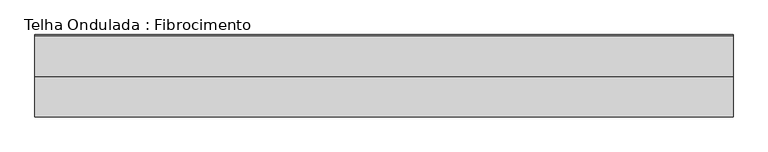
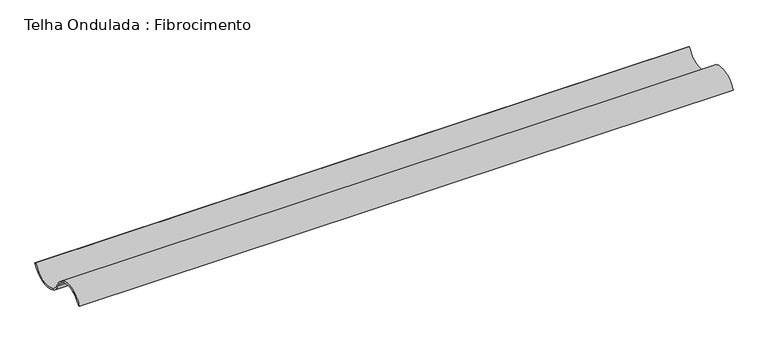
"""IFC4 building model written with IfcOpenShell, lengths in millimetres: beam geometry, Telha Ondulada : Fibrocimento."""

from ifc_helpers import new_model, si_unit, point, frame, frame_2d, origin, place, context, project, spatial, polyline, circle_curve, trimmed, segment, composite_curve, outline, extrude, source, transform, mapped, element, save


def telha_ondulada_fibrocimento_69359d52(model_context):
    return source(origin(), model_context, "Body", "SweptSolid", [
        extrude(outline(composite_curve([segment(trimmed(circle_curve(frame_2d((68.3970135, 71.7939461)), 66.7939461), [point((8.3970135, 42.4437972))], [point((128.3970135, 42.4437972))], True, "CARTESIAN"), True, "CONTINUOUS"), segment(polyline([(128.3970135, 42.4437972), (132.8884385, 40.2467307)]), True, "CONTINUOUS"), segment(trimmed(circle_curve(frame_2d((68.3970135, 71.7939461)), 71.7939461), [point((132.8884385, 40.2467307))], [point((3.9055884, 40.2467307))], False, "CARTESIAN"), True, "CONTINUOUS"), segment(trimmed(circle_curve(frame_2d((-51.6029865, 13.0936483)), 61.7939461), [point((3.9055884, 40.2467307))], [point((-107.1115615, 40.2467307))], True, "CARTESIAN"), True, "CONTINUOUS"), segment(polyline([(-107.1115615, 40.2467307), (-111.6029865, 42.4437972)]), True, "CONTINUOUS"), segment(trimmed(circle_curve(frame_2d((-51.6029865, 13.0936483)), 66.7939461), [point((-111.6029865, 42.4437972))], [point((8.3970135, 42.4437972))], False, "CARTESIAN"), True, "CONTINUOUS")], self_intersect=False)), frame((-1038.2805783, 0.0, 0.0), z_axis=(1.0, 0.0, 0.0), x_axis=(0.0, 1.0, 0.0)), (0.0, 0.0, 1.0), 2076.5611566),
    ])


if __name__ == "__main__":
    model = new_model("IFC4")
    model_context = context("Model", 3, world=origin())
    ifc_project = project(units=[si_unit("LENGTHUNIT", "METRE", prefix="MILLI")], contexts=[model_context])
    site = spatial("IfcSite", under=ifc_project)
    building = spatial("IfcBuilding", under=site)
    placement = place(None, origin())
    telha_ondulada_fibrocimento_shape = telha_ondulada_fibrocimento_69359d52(model_context)
    element("IfcBeam", 1, ObjectType="Telha Ondulada : Fibrocimento", at=placement, inside=building, context=model_context, shape_type="MappedRepresentation", body=[
        mapped(telha_ondulada_fibrocimento_shape, transform((0.0, 0.0, 0.0), x_axis=(1.0, 0.0, 0.0), y_axis=(0.0, 1.0, 0.0), z_axis=(0.0, 0.0, 1.0))),
    ])
    save(model, "model.ifc")

# Revit data of these elements
# Type "Telha Ondulada : Fibrocimento"
#   Description = "TELHA ONDULADA FIBROCIMENTO"
#   Cost = 5
#   Length [instance default] = 1.524 m
#   b = 0.07 m
#   h = 0.16 m
#   Structural Material = .TELHA DE FIBROCIMENTO
#   Assembly Code = ""
# Element 1 (IfcBeam, "Telha Ondulada : Fibrocimento")
#   Materials on its faces: ".TELHA DE FIBROCIMENTO"
# Materials
#   ".TELHA DE FIBROCIMENTO": class "CC_TELHADO", colour RGB 77 77 76, transparency 0, Description = "TELHA ONDULADA FIBROCIMENTO", Cost = 0
